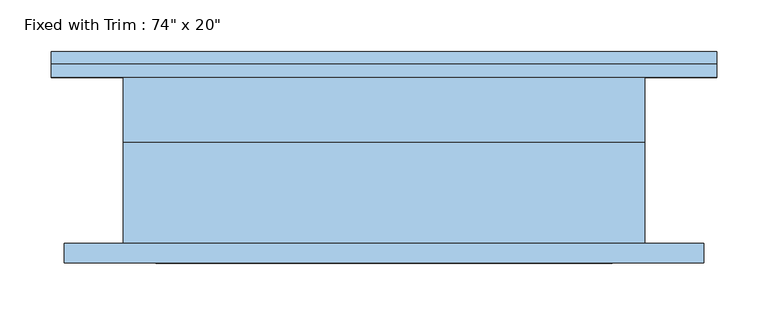
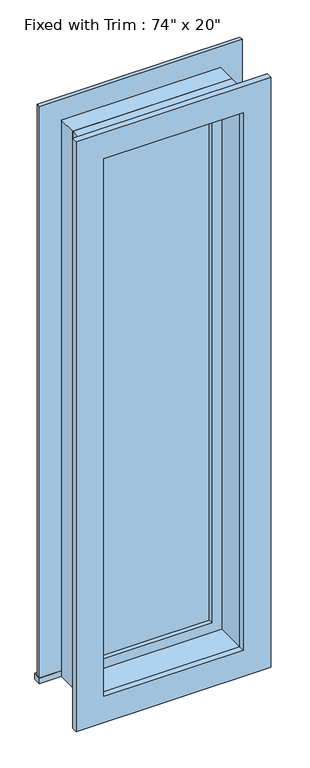
"""IFC4 building model written with IfcOpenShell, lengths in millimetres: window geometry."""

from ifc_helpers import new_model, si_unit, frame, origin, place, context, project, spatial, polyline, outline, extrude, source, transform, mapped, element, save


def window_deeb26d8(model_context):
    return source(origin(), model_context, "Body", "SweptSolid", [
        extrude(outline(polyline([(-361.95, 106.3625), (285.75, 106.3625), (285.75, 80.9625), (-361.95, 80.9625), (-361.95, 106.3625)])), frame((0.0, 0.0, 914.4), z_axis=(0.0, 0.0, 1.0), x_axis=(1.0, 0.0, 0.0)), (0.0, 0.0, 1.0), 19.05),
        extrude(outline(polyline([(2774.95, -273.05), (2774.95, 196.85), (933.45, 196.85), (933.45, 285.75), (2863.85, 285.75), (2863.85, -361.95), (933.45, -361.95), (933.45, -273.05), (2774.95, -273.05)])), frame((0.0, 80.9625, 0.0), z_axis=(0.0, 1.0, 0.0), x_axis=(0.0, 0.0, 1.0)), (0.0, 0.0, 1.0), 12.7),
        extrude(outline(polyline([(2851.15, 273.05), (2851.15, -349.25), (857.25, -349.25), (857.25, 273.05), (2851.15, 273.05)]), holes=[polyline([(2762.25, 184.15), (946.15, 184.15), (946.15, -260.35), (2762.25, -260.35), (2762.25, 184.15)])]), frame((0.0, -100.0125, 0.0), z_axis=(0.0, 1.0, 0.0), x_axis=(0.0, 0.0, 1.0)), (0.0, 0.0, 1.0), 19.05),
        extrude(outline(polyline([(152.4, 33.3375), (-228.6, 33.3375), (-228.6, 46.0375), (152.4, 46.0375), (152.4, 33.3375)])), frame((0.0, 0.0, 977.9), z_axis=(0.0, 0.0, 1.0), x_axis=(1.0, 0.0, 0.0)), (0.0, 0.0, 1.0), 1752.6),
        extrude(outline(polyline([(2774.95, -273.05), (933.45, -273.05), (933.45, 196.85), (2774.95, 196.85), (2774.95, -273.05)]), holes=[polyline([(2730.5, -228.6), (2730.5, 152.4), (977.9, 152.4), (977.9, -228.6), (2730.5, -228.6)])]), frame((0.0, 17.4625, 0.0), z_axis=(0.0, 1.0, 0.0), x_axis=(0.0, 0.0, 1.0)), (0.0, 0.0, 1.0), 44.45),
        extrude(outline(polyline([(2794.0, -292.1), (914.4, -292.1), (914.4, 215.9), (2794.0, 215.9), (2794.0, -292.1)]), holes=[polyline([(2762.25, -260.35), (2762.25, 184.15), (946.15, 184.15), (946.15, -260.35), (2762.25, -260.35)])]), frame((0.0, -80.9625, 0.0), z_axis=(0.0, 1.0, 0.0), x_axis=(0.0, 0.0, 1.0)), (0.0, 0.0, 1.0), 98.425),
        extrude(outline(polyline([(2794.0, 215.9), (2794.0, -292.1), (914.4, -292.1), (914.4, 215.9), (2794.0, 215.9)]), holes=[polyline([(2774.95, 196.85), (933.45, 196.85), (933.45, -273.05), (2774.95, -273.05), (2774.95, 196.85)])]), frame((0.0, 17.4625, 0.0), z_axis=(0.0, 1.0, 0.0), x_axis=(0.0, 0.0, 1.0)), (0.0, 0.0, 1.0), 63.5),
    ])


if __name__ == "__main__":
    model = new_model("IFC4")
    model_context = context("Model", 3, world=origin())
    ifc_project = project(units=[si_unit("LENGTHUNIT", "METRE", prefix="MILLI")], contexts=[model_context])
    site = spatial("IfcSite", under=ifc_project)
    building = spatial("IfcBuilding", under=site)
    placement = place(None, origin())
    window_shape = window_deeb26d8(model_context)
    element("IfcWindow", 1, ObjectType="Fixed with Trim : 74\" x 20\"", at=placement, inside=building, context=model_context, shape_type="MappedRepresentation", body=[
        mapped(window_shape, transform((0.0, 0.0, 0.0), x_axis=(1.0, 0.0, 0.0), y_axis=(0.0, 1.0, 0.0), z_axis=(0.0, 0.0, 1.0))),
    ])
    save(model, "model.ifc")

# Revit data of these elements
# Type "Fixed with Trim : 74\" x 20\""
#   Type Mark = "59"
#   COBie.Type.CreatedBy = "doug.wood@us.ibm.com"
#   COBie.Type.CreatedOn = "2016-04-14T02:07:26"
#   COBie.Type.Name = "Windows_Fixed with Trim_74\" x 20\"_59"
#   COBie.Type.Category = "23-30 20 17 11 : Fixed Windows"
#   COBie.Type.Description = "Fixed with Trim_74\" x 20\""
#   COBie.Type.Manufacturer = ""
#   COBie.Type.ModelNumber = ""
#   Construction Type Id = "GSP4R"
#   Assembly Code = "B2020100"
#   Analytic Construction = "1/8 in Pilkington single glazing"
#   COBie.Type.ReplacementCost = 0
#   Visual Light Transmittance = 0.9
#   Solar Heat Gain Coefficient = 0.78
#   Heat Transfer Coefficient (U) = 3.6886 W/(m²·K)
#   Height = 6' - 2"
#   Default Sill Height = 3' - 0"
#   Trim Projection - Ext. = 0' - 0 1/2"
#   Trim Projection - Int. = 0' - 0 3/4"
#   Trim Width - Exterior = 0' - 3 1/2"
#   Trim Width - Interior = 0' - 3 1/2"
#   Width = 1' - 8"
#   Window Inset = 0' - 0 3/4"
#   COBie.Type = no
#   Glass Pane Material = Glass
#   Sash Material = Sash - White
#   Trim Exterior Material = Trim - White
#   Trim Interior Material = Trim - White
#   Wall Closure = (empty or 0)
# Element 1 (IfcWindow, "Fixed with Trim : 74\" x 20\"")
#   Materials on its faces: "Sash - White", "Trim - White", "Glass"
# Materials
#   "Glass": class "Glass", colour RGB 0 128 192, transparency 0.75, Description = "Soda Lime Glass", Cost = 0
#   "Sash - White": class "Wood", colour RGB 255 255 255, transparency 0, Cost = 0
#   "Trim - White": class "Wood", colour RGB 255 255 255, transparency 0, Cost = 0
